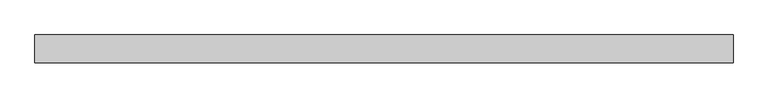
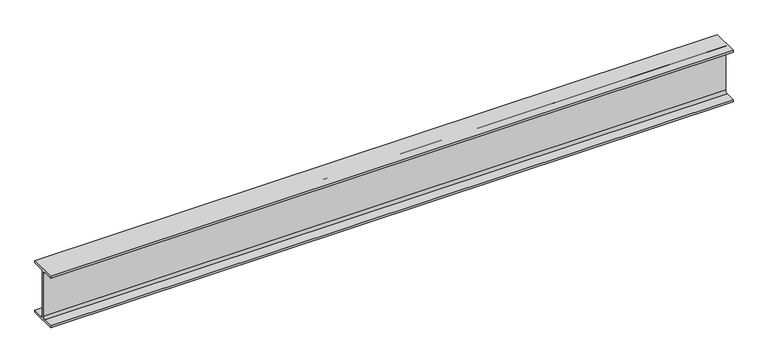
"""IFC4 building model written with IfcOpenShell, lengths in millimetres: beam geometry, 0912_Steel Framing_H-KSD3502 : H_SB_ASB_H-250x125x6x9."""

import ifcopenshell
import ifcopenshell.guid

model = None  # the IFC model being written
_history = None  # IfcOwnerHistory: only IFC2X3 demands one
_inside = {}  # id of a spatial element -> (the spatial element, [elements in it])
_under = {}  # id of a project, library or spatial element -> (it, [spatial elements below it])
_declared = {}  # id of a project -> (the project, [libraries it declares])
_typed = {}  # id of a type object -> (the type object, [elements of that type])
_made_of = {}  # id of a material, layer set ... -> (it, [elements and type objects made of it])


def new_model(schema):
    """Start an empty IFC model of exactly this schema.

    Asked for "IFC4X3", IfcOpenShell would pick the latest addendum, in which some entities
    have other attributes; the version numbers below select the first issue.
    IFC2X3 requires an IfcOwnerHistory on every rooted entity: one is made here for all.
    """
    global model, _history
    if schema == "IFC4X3":
        model = ifcopenshell.file(schema_version=(4, 3, 0, 0))
    else:
        model = ifcopenshell.file(schema=schema)
    _inside.clear()
    _under.clear()
    _declared.clear()
    _typed.clear()
    _made_of.clear()
    _history = None
    if model.schema == "IFC2X3":
        org = make("IfcOrganization", Name="unknown")
        user = make(
            "IfcPersonAndOrganization",
            ThePerson=make("IfcPerson", FamilyName="unknown"),
            TheOrganization=org,
        )
        app = make(
            "IfcApplication",
            ApplicationDeveloper=org,
            Version="unknown",
            ApplicationFullName="unknown",
            ApplicationIdentifier="unknown",
        )
        _history = make(
            "IfcOwnerHistory",
            OwningUser=user,
            OwningApplication=app,
            ChangeAction="ADDED",
            CreationDate=0,
        )
    return model


def make(cls, **values):
    """One entity of the class cls with the attributes given. An attribute that is None is left unset."""
    return model.create_entity(
        cls, **{name: value for name, value in values.items() if value is not None}
    )


def rooted(cls, **values):
    """An entity with a GlobalId (a new one), such as an element, a storey or a relation."""
    return make(cls, GlobalId=ifcopenshell.guid.new(), OwnerHistory=_history, **values)


def si_unit(unit_type, name, prefix=None):
    """IfcSIUnit, for example si_unit("LENGTHUNIT", "METRE", prefix="MILLI")."""
    return make("IfcSIUnit", UnitType=unit_type, Prefix=prefix, Name=name)


def assignment(units):
    """IfcUnitAssignment: the units of a project."""
    return None if units is None else make("IfcUnitAssignment", Units=units)


def point(xyz):
    """IfcCartesianPoint."""
    return None if xyz is None else make("IfcCartesianPoint", Coordinates=xyz)


def direction(xyz):
    """IfcDirection."""
    return None if xyz is None else make("IfcDirection", DirectionRatios=xyz)


def frame(location, z_axis=None, x_axis=None):
    """IfcAxis2Placement3D, a coordinate frame: its origin and axes. An axis left out is left unset."""
    return make(
        "IfcAxis2Placement3D",
        Location=point(location),
        Axis=direction(z_axis),
        RefDirection=direction(x_axis),
    )


def frame_2d(location, x_axis=None):
    """IfcAxis2Placement2D, a coordinate frame in the plane: its origin and x axis."""
    return make(
        "IfcAxis2Placement2D", Location=point(location), RefDirection=direction(x_axis)
    )


def origin():
    """The frame at (0, 0, 0) with its axes left unset."""
    return frame((0.0, 0.0, 0.0))


def place(relative_to, where):
    """IfcLocalPlacement: puts the frame where relative to a parent placement (None: the world)."""
    return make(
        "IfcLocalPlacement", PlacementRelTo=relative_to, RelativePlacement=where
    )


def context(
    kind, dimensions, precision=None, world=None, true_north=None, identifier=None
):
    """IfcGeometricRepresentationContext, for example the 3D "Model" context."""
    return make(
        "IfcGeometricRepresentationContext",
        ContextIdentifier=identifier,
        ContextType=kind,
        CoordinateSpaceDimension=dimensions,
        Precision=precision,
        WorldCoordinateSystem=world,
        TrueNorth=true_north,
    )


def project(units=None, contexts=None):
    """IfcProject with its units and contexts."""
    return rooted(
        "IfcProject",
        Name="project",
        RepresentationContexts=contexts,
        UnitsInContext=assignment(units),
    )


def spatial(cls, under=None, at=None, **own):
    """A site, building, storey or space (cls), placed at a placement, below another one or the project."""
    s = rooted(cls, ObjectPlacement=at, **own)
    if under is not None:
        _under.setdefault(under.id(), (under, []))[1].append(s)
    return s


def polyline(points):
    """IfcPolyline through the points."""
    return make("IfcPolyline", Points=[point(p) for p in points])


def circle_curve(where, radius):
    """IfcCircle in the frame where."""
    return make("IfcCircle", Position=where, Radius=radius)


def trimmed(basis, trim1, trim2, sense, master):
    """IfcTrimmedCurve: the piece of a basis curve between two trims."""
    return make(
        "IfcTrimmedCurve",
        BasisCurve=basis,
        Trim1=trim1,
        Trim2=trim2,
        SenseAgreement=sense,
        MasterRepresentation=master,
    )


def segment(curve, same_sense, transition):
    """IfcCompositeCurveSegment."""
    return make(
        "IfcCompositeCurveSegment",
        Transition=transition,
        SameSense=same_sense,
        ParentCurve=curve,
    )


def composite_curve(segments, self_intersect=None):
    """IfcCompositeCurve: segments joined end to end."""
    return make("IfcCompositeCurve", Segments=segments, SelfIntersect=self_intersect)


def outline(outer, holes=None, kind="AREA"):
    """IfcArbitraryClosedProfileDef: a profile drawn as a closed curve; with holes, ...WithVoids."""
    if holes is None:
        return make("IfcArbitraryClosedProfileDef", ProfileType=kind, OuterCurve=outer)
    return make(
        "IfcArbitraryProfileDefWithVoids",
        ProfileType=kind,
        OuterCurve=outer,
        InnerCurves=holes,
    )


def extrude(swept, where, along, depth):
    """IfcExtrudedAreaSolid: the profile swept, set in the frame where, extruded along a direction by depth."""
    return make(
        "IfcExtrudedAreaSolid",
        SweptArea=swept,
        Position=where,
        ExtrudedDirection=direction(along),
        Depth=depth,
    )


def shape(context_of_items, identifier, shape_type, items):
    """IfcShapeRepresentation: the items that make up one representation, for example the "Body"."""
    return make(
        "IfcShapeRepresentation",
        ContextOfItems=context_of_items,
        RepresentationIdentifier=identifier,
        RepresentationType=shape_type,
        Items=items,
    )


def source(mapping_origin, context_of_items, identifier, shape_type, items):
    """IfcRepresentationMap: a shape defined once, which mapped items show again and again."""
    return make(
        "IfcRepresentationMap",
        MappingOrigin=mapping_origin,
        MappedRepresentation=shape(context_of_items, identifier, shape_type, items),
    )


def transform(
    local_origin,
    x_axis=None,
    y_axis=None,
    z_axis=None,
    scale=None,
    scale2=None,
    scale3=None,
    uniform=True,
):
    """IfcCartesianTransformationOperator3D, or its non-uniform kind. x_axis, y_axis, z_axis: its Axis1, 2, 3."""
    if uniform:
        return make(
            "IfcCartesianTransformationOperator3D",
            Axis1=direction(x_axis),
            Axis2=direction(y_axis),
            LocalOrigin=point(local_origin),
            Scale=scale,
            Axis3=direction(z_axis),
        )
    return make(
        "IfcCartesianTransformationOperator3DnonUniform",
        Axis1=direction(x_axis),
        Axis2=direction(y_axis),
        LocalOrigin=point(local_origin),
        Scale=scale,
        Axis3=direction(z_axis),
        Scale2=scale2,
        Scale3=scale3,
    )


def mapped(mapping_source, mapping_target):
    """IfcMappedItem: shows the shape of a source again, moved by a transform."""
    return make(
        "IfcMappedItem", MappingSource=mapping_source, MappingTarget=mapping_target
    )


def made_of(thing, what):
    """Note that an element or type object is made of a material, layer set ...; save() writes the relation."""
    if what is not None:
        _made_of.setdefault(what.id(), (what, []))[1].append(thing)
    return thing


def element(
    cls,
    number,
    at=None,
    inside=None,
    cuts=None,
    type_object=None,
    material=None,
    context=None,
    identifier="Body",
    shape_type=None,
    held_by="IfcProductDefinitionShape",
    body=None,
    shapes=None,
    **own,
):
    """One element of the class cls, such as IfcWall. Its Tag is "e" and its number.

    at: its placement. inside: the storey or other place that contains it. cuts: it is an
    opening in that element (IfcRelVoidsElement). A single representation is given by context,
    identifier, shape_type and body (its items); several are given by shapes. held_by: the class
    of the entity that holds the representations. save() writes the other relations.
    """
    e = rooted(cls, Tag="e%d" % number, ObjectPlacement=at, **own)
    if body is not None:
        shapes = [shape(context, identifier, shape_type, body)]
    if shapes is not None:
        e.Representation = make(held_by, Representations=shapes)
    if inside is not None:
        _inside.setdefault(inside.id(), (inside, []))[1].append(e)
    if cuts is not None:
        rooted(
            "IfcRelVoidsElement", RelatingBuildingElement=cuts, RelatedOpeningElement=e
        )
    if type_object is not None:
        _typed.setdefault(type_object.id(), (type_object, []))[1].append(e)
    return made_of(e, material)


def aggregate(whole, parts):
    """IfcRelAggregates: a whole, such as a stair, and the parts it consists of."""
    return rooted("IfcRelAggregates", RelatingObject=whole, RelatedObjects=parts)


def save(model, path):
    """Write the relations noted so far, then the file.

    IfcRelAggregates (storeys below a building ...), IfcRelContainedInSpatialStructure (elements
    in a storey), IfcRelDefinesByType, IfcRelAssociatesMaterial and IfcRelDeclares: one each for
    every whole, place, type object, material and project.
    """
    for whole, parts in _under.values():
        aggregate(whole, parts)
    for where, things in _inside.values():
        rooted(
            "IfcRelContainedInSpatialStructure",
            RelatedElements=things,
            RelatingStructure=where,
        )
    for kind, things in _typed.values():
        rooted("IfcRelDefinesByType", RelatedObjects=things, RelatingType=kind)
    for what, things in _made_of.values():
        rooted("IfcRelAssociatesMaterial", RelatedObjects=things, RelatingMaterial=what)
    for by, libraries in _declared.values():
        rooted("IfcRelDeclares", RelatingContext=by, RelatedDefinitions=libraries)
    model.write(path)


def beam_cd7e6579(model_context):
    return source(origin(), model_context, "Body", "SweptSolid", [
        extrude(outline(composite_curve([segment(polyline([(62.5, -116.0), (62.5, -125.0), (-62.5, -125.0), (-62.5, -116.0), (-15.0, -116.0)]), True, "CONTINUOUS"), segment(trimmed(circle_curve(frame_2d((-15.0, -104.0)), 12.0), [point((-15.0, -116.0))], [point((-3.0, -104.0))], True, "CARTESIAN"), True, "CONTINUOUS"), segment(polyline([(-3.0, -104.0), (-3.0, 104.0)]), True, "CONTINUOUS"), segment(trimmed(circle_curve(frame_2d((-15.0, 104.0)), 12.0), [point((-3.0, 104.0))], [point((-15.0, 116.0))], True, "CARTESIAN"), True, "CONTINUOUS"), segment(polyline([(-15.0, 116.0), (-62.5, 116.0), (-62.5, 125.0), (62.5, 125.0), (62.5, 116.0), (15.0, 116.0)]), True, "CONTINUOUS"), segment(trimmed(circle_curve(frame_2d((15.0, 104.0)), 12.0), [point((15.0, 116.0))], [point((3.0, 104.0))], True, "CARTESIAN"), True, "CONTINUOUS"), segment(polyline([(3.0, 104.0), (3.0, -104.0)]), True, "CONTINUOUS"), segment(trimmed(circle_curve(frame_2d((15.0, -104.0)), 12.0), [point((3.0, -104.0))], [point((15.0, -116.0))], True, "CARTESIAN"), True, "CONTINUOUS"), segment(polyline([(15.0, -116.0), (62.5, -116.0)]), True, "CONTINUOUS")], self_intersect=False)), frame((-1654.8000435, 0.0, 0.0), z_axis=(1.0, 0.0, 0.0), x_axis=(0.0, 1.0, 0.0)), (0.0, 0.0, 1.0), 3149.2888185),
    ])


if __name__ == "__main__":
    model = new_model("IFC4")
    model_context = context("Model", 3, world=origin())
    ifc_project = project(units=[si_unit("LENGTHUNIT", "METRE", prefix="MILLI")], contexts=[model_context])
    site = spatial("IfcSite", under=ifc_project)
    building = spatial("IfcBuilding", under=site)
    placement = place(None, origin())
    beam_shape = beam_cd7e6579(model_context)
    element("IfcBeam", 1, ObjectType="0912_Steel Framing_H-KSD3502 : H_SB_ASB_H-250x125x6x9", at=placement, inside=building, context=model_context, shape_type="MappedRepresentation", body=[
        mapped(beam_shape, transform((0.0, 0.0, 0.0), x_axis=(1.0, 0.0, 0.0), y_axis=(0.0, 1.0, 0.0), z_axis=(0.0, 0.0, 1.0))),
    ])
    save(model, "model.ifc")

# Revit data of these elements
# Type "0912_Steel Framing_H-KSD3502 : H_SB_ASB_H-250x125x6x9"
#   H_WM Code_1 = "S01AA003-00001 | Main Steel Structure Fabrication Work | Shelter/Building | Light Steel - Standard (30KG/M>Weight) | Material: (   )"
#   H_WM Code_2 = "S03AA029-00001 | Main Steel Structure Erection Work | Shelter/Building | Light Steel (30KG/M>Weight) | Material: (   )"
#   H_WM Code_3 = "S01AA010-00001 | Main Steel Structure Fabrication Work | Shelter/Building | Steel Painting/Coating | for Non-Fireproofed Steel Surface, Surface Preparation, Primer, Second & Final Coat | Material: (   )"
#   H_Q'ty Cal Type Tag = "SB-Q2"
#   Width = 12.5 cm
#   Web Thickness = 0.6 cm
#   Web Fillet = 1.2 cm
#   Warping Constant = 42539.8 cm⁶
#   W = 0
#   Torsional Moment of Inertia = 7.8102 cm⁴
#   Section Area = 37.66 cm²
#   Plastic Modulus weak axis = 73.1 cm³
#   Plastic Modulus strong axis = 366.0 cm³
#   Perimeter = 0.97 m²/m
#   Nominal Weight = 29.60 kgf/m
#   Moment of Inertia weak axis = 294.00 cm⁴
#   Moment of Inertia strong axis = 4050.00 cm⁴
#   Height = 25.0 cm
#   Flange Thickness = 0.9 cm
#   Elastic Modulus weak axis = 47.0 cm³
#   Elastic Modulus strong axis = 324.0 cm³
#   Centroid Vertical = 12.5 cm
#   Centroid Horizontal = 6.25 cm
#   Ix = 40500000
#   Length [instance default] = 1.5240 m
#   Zx = 366000
#   b = 0.1250 m
#   h = 0.2500 m
#   r = 0.0120 m
#   s = 0.0060 m
#   t = 0.0090 m
#   A = 0.003766 m²
#   Structural Material [instance default] = Steel, 45-345
#   Assembly Code = ""
# Element 1 (IfcBeam, "0912_Steel Framing_H-KSD3502 : H_SB_ASB_H-250x125x6x9")
#   Structural Material = none
# Materials
#   "Steel, 45-345": class "Metal", colour RGB 189 187 185, transparency 0, Description = "Steel 345 MPa", Cost = 0
